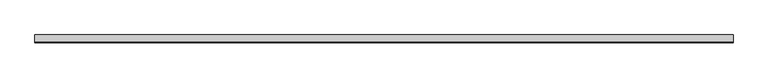
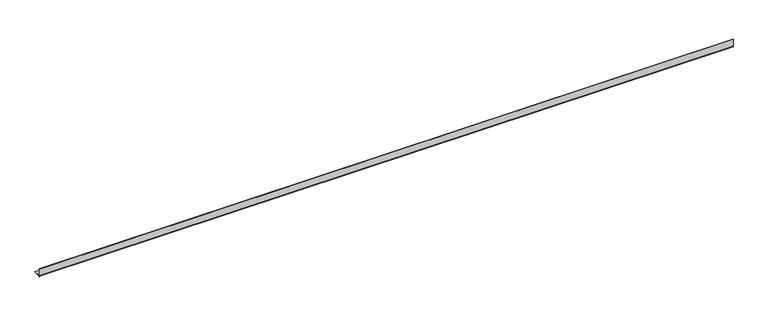
"""IFC4 building model written with IfcOpenShell, lengths in millimetres: proxy geometry, Metal profile010 3100 : Metal profile010 3100."""

import ifcopenshell
import ifcopenshell.guid

model = None  # the IFC model being written
_history = None  # IfcOwnerHistory: only IFC2X3 demands one
_inside = {}  # id of a spatial element -> (the spatial element, [elements in it])
_under = {}  # id of a project, library or spatial element -> (it, [spatial elements below it])
_declared = {}  # id of a project -> (the project, [libraries it declares])
_typed = {}  # id of a type object -> (the type object, [elements of that type])
_made_of = {}  # id of a material, layer set ... -> (it, [elements and type objects made of it])


def new_model(schema):
    """Start an empty IFC model of exactly this schema.

    Asked for "IFC4X3", IfcOpenShell would pick the latest addendum, in which some entities
    have other attributes; the version numbers below select the first issue.
    IFC2X3 requires an IfcOwnerHistory on every rooted entity: one is made here for all.
    """
    global model, _history
    if schema == "IFC4X3":
        model = ifcopenshell.file(schema_version=(4, 3, 0, 0))
    else:
        model = ifcopenshell.file(schema=schema)
    _inside.clear()
    _under.clear()
    _declared.clear()
    _typed.clear()
    _made_of.clear()
    _history = None
    if model.schema == "IFC2X3":
        org = make("IfcOrganization", Name="unknown")
        user = make(
            "IfcPersonAndOrganization",
            ThePerson=make("IfcPerson", FamilyName="unknown"),
            TheOrganization=org,
        )
        app = make(
            "IfcApplication",
            ApplicationDeveloper=org,
            Version="unknown",
            ApplicationFullName="unknown",
            ApplicationIdentifier="unknown",
        )
        _history = make(
            "IfcOwnerHistory",
            OwningUser=user,
            OwningApplication=app,
            ChangeAction="ADDED",
            CreationDate=0,
        )
    return model


def make(cls, **values):
    """One entity of the class cls with the attributes given. An attribute that is None is left unset."""
    return model.create_entity(
        cls, **{name: value for name, value in values.items() if value is not None}
    )


def rooted(cls, **values):
    """An entity with a GlobalId (a new one), such as an element, a storey or a relation."""
    return make(cls, GlobalId=ifcopenshell.guid.new(), OwnerHistory=_history, **values)


def si_unit(unit_type, name, prefix=None):
    """IfcSIUnit, for example si_unit("LENGTHUNIT", "METRE", prefix="MILLI")."""
    return make("IfcSIUnit", UnitType=unit_type, Prefix=prefix, Name=name)


def assignment(units):
    """IfcUnitAssignment: the units of a project."""
    return None if units is None else make("IfcUnitAssignment", Units=units)


def point(xyz):
    """IfcCartesianPoint."""
    return None if xyz is None else make("IfcCartesianPoint", Coordinates=xyz)


def direction(xyz):
    """IfcDirection."""
    return None if xyz is None else make("IfcDirection", DirectionRatios=xyz)


def frame(location, z_axis=None, x_axis=None):
    """IfcAxis2Placement3D, a coordinate frame: its origin and axes. An axis left out is left unset."""
    return make(
        "IfcAxis2Placement3D",
        Location=point(location),
        Axis=direction(z_axis),
        RefDirection=direction(x_axis),
    )


def frame_2d(location, x_axis=None):
    """IfcAxis2Placement2D, a coordinate frame in the plane: its origin and x axis."""
    return make(
        "IfcAxis2Placement2D", Location=point(location), RefDirection=direction(x_axis)
    )


def origin():
    """The frame at (0, 0, 0) with its axes left unset."""
    return frame((0.0, 0.0, 0.0))


def place(relative_to, where):
    """IfcLocalPlacement: puts the frame where relative to a parent placement (None: the world)."""
    return make(
        "IfcLocalPlacement", PlacementRelTo=relative_to, RelativePlacement=where
    )


def context(
    kind, dimensions, precision=None, world=None, true_north=None, identifier=None
):
    """IfcGeometricRepresentationContext, for example the 3D "Model" context."""
    return make(
        "IfcGeometricRepresentationContext",
        ContextIdentifier=identifier,
        ContextType=kind,
        CoordinateSpaceDimension=dimensions,
        Precision=precision,
        WorldCoordinateSystem=world,
        TrueNorth=true_north,
    )


def project(units=None, contexts=None):
    """IfcProject with its units and contexts."""
    return rooted(
        "IfcProject",
        Name="project",
        RepresentationContexts=contexts,
        UnitsInContext=assignment(units),
    )


def spatial(cls, under=None, at=None, **own):
    """A site, building, storey or space (cls), placed at a placement, below another one or the project."""
    s = rooted(cls, ObjectPlacement=at, **own)
    if under is not None:
        _under.setdefault(under.id(), (under, []))[1].append(s)
    return s


def polyline(points):
    """IfcPolyline through the points."""
    return make("IfcPolyline", Points=[point(p) for p in points])


def circle_curve(where, radius):
    """IfcCircle in the frame where."""
    return make("IfcCircle", Position=where, Radius=radius)


def trimmed(basis, trim1, trim2, sense, master):
    """IfcTrimmedCurve: the piece of a basis curve between two trims."""
    return make(
        "IfcTrimmedCurve",
        BasisCurve=basis,
        Trim1=trim1,
        Trim2=trim2,
        SenseAgreement=sense,
        MasterRepresentation=master,
    )


def segment(curve, same_sense, transition):
    """IfcCompositeCurveSegment."""
    return make(
        "IfcCompositeCurveSegment",
        Transition=transition,
        SameSense=same_sense,
        ParentCurve=curve,
    )


def composite_curve(segments, self_intersect=None):
    """IfcCompositeCurve: segments joined end to end."""
    return make("IfcCompositeCurve", Segments=segments, SelfIntersect=self_intersect)


def outline(outer, holes=None, kind="AREA"):
    """IfcArbitraryClosedProfileDef: a profile drawn as a closed curve; with holes, ...WithVoids."""
    if holes is None:
        return make("IfcArbitraryClosedProfileDef", ProfileType=kind, OuterCurve=outer)
    return make(
        "IfcArbitraryProfileDefWithVoids",
        ProfileType=kind,
        OuterCurve=outer,
        InnerCurves=holes,
    )


def extrude(swept, where, along, depth):
    """IfcExtrudedAreaSolid: the profile swept, set in the frame where, extruded along a direction by depth."""
    return make(
        "IfcExtrudedAreaSolid",
        SweptArea=swept,
        Position=where,
        ExtrudedDirection=direction(along),
        Depth=depth,
    )


def shape(context_of_items, identifier, shape_type, items):
    """IfcShapeRepresentation: the items that make up one representation, for example the "Body"."""
    return make(
        "IfcShapeRepresentation",
        ContextOfItems=context_of_items,
        RepresentationIdentifier=identifier,
        RepresentationType=shape_type,
        Items=items,
    )


def source(mapping_origin, context_of_items, identifier, shape_type, items):
    """IfcRepresentationMap: a shape defined once, which mapped items show again and again."""
    return make(
        "IfcRepresentationMap",
        MappingOrigin=mapping_origin,
        MappedRepresentation=shape(context_of_items, identifier, shape_type, items),
    )


def transform(
    local_origin,
    x_axis=None,
    y_axis=None,
    z_axis=None,
    scale=None,
    scale2=None,
    scale3=None,
    uniform=True,
):
    """IfcCartesianTransformationOperator3D, or its non-uniform kind. x_axis, y_axis, z_axis: its Axis1, 2, 3."""
    if uniform:
        return make(
            "IfcCartesianTransformationOperator3D",
            Axis1=direction(x_axis),
            Axis2=direction(y_axis),
            LocalOrigin=point(local_origin),
            Scale=scale,
            Axis3=direction(z_axis),
        )
    return make(
        "IfcCartesianTransformationOperator3DnonUniform",
        Axis1=direction(x_axis),
        Axis2=direction(y_axis),
        LocalOrigin=point(local_origin),
        Scale=scale,
        Axis3=direction(z_axis),
        Scale2=scale2,
        Scale3=scale3,
    )


def mapped(mapping_source, mapping_target):
    """IfcMappedItem: shows the shape of a source again, moved by a transform."""
    return make(
        "IfcMappedItem", MappingSource=mapping_source, MappingTarget=mapping_target
    )


def made_of(thing, what):
    """Note that an element or type object is made of a material, layer set ...; save() writes the relation."""
    if what is not None:
        _made_of.setdefault(what.id(), (what, []))[1].append(thing)
    return thing


def element(
    cls,
    number,
    at=None,
    inside=None,
    cuts=None,
    type_object=None,
    material=None,
    context=None,
    identifier="Body",
    shape_type=None,
    held_by="IfcProductDefinitionShape",
    body=None,
    shapes=None,
    **own,
):
    """One element of the class cls, such as IfcWall. Its Tag is "e" and its number.

    at: its placement. inside: the storey or other place that contains it. cuts: it is an
    opening in that element (IfcRelVoidsElement). A single representation is given by context,
    identifier, shape_type and body (its items); several are given by shapes. held_by: the class
    of the entity that holds the representations. save() writes the other relations.
    """
    e = rooted(cls, Tag="e%d" % number, ObjectPlacement=at, **own)
    if body is not None:
        shapes = [shape(context, identifier, shape_type, body)]
    if shapes is not None:
        e.Representation = make(held_by, Representations=shapes)
    if inside is not None:
        _inside.setdefault(inside.id(), (inside, []))[1].append(e)
    if cuts is not None:
        rooted(
            "IfcRelVoidsElement", RelatingBuildingElement=cuts, RelatedOpeningElement=e
        )
    if type_object is not None:
        _typed.setdefault(type_object.id(), (type_object, []))[1].append(e)
    return made_of(e, material)


def aggregate(whole, parts):
    """IfcRelAggregates: a whole, such as a stair, and the parts it consists of."""
    return rooted("IfcRelAggregates", RelatingObject=whole, RelatedObjects=parts)


def save(model, path):
    """Write the relations noted so far, then the file.

    IfcRelAggregates (storeys below a building ...), IfcRelContainedInSpatialStructure (elements
    in a storey), IfcRelDefinesByType, IfcRelAssociatesMaterial and IfcRelDeclares: one each for
    every whole, place, type object, material and project.
    """
    for whole, parts in _under.values():
        aggregate(whole, parts)
    for where, things in _inside.values():
        rooted(
            "IfcRelContainedInSpatialStructure",
            RelatedElements=things,
            RelatingStructure=where,
        )
    for kind, things in _typed.values():
        rooted("IfcRelDefinesByType", RelatedObjects=things, RelatingType=kind)
    for what, things in _made_of.values():
        rooted("IfcRelAssociatesMaterial", RelatedObjects=things, RelatingMaterial=what)
    for by, libraries in _declared.values():
        rooted("IfcRelDeclares", RelatingContext=by, RelatedDefinitions=libraries)
    model.write(path)


def generic_models_2c1d3a63(model_context):
    return source(origin(), model_context, "Body", "SweptSolid", [
        extrude(outline(composite_curve([segment(polyline([(10261.8870729, 42910.4253714), (10261.8870729, 42889.2721875), (10283.0402569, 42889.2721875), (10283.0402569, 42887.9921875), (10262.1373472, 42887.9921875)]), True, "CONTINUOUS"), segment(trimmed(circle_curve(frame_2d((10261.2470729, 42888.6321875)), 1.0964434), [point((10262.1373472, 42887.9921875))], [point((10260.6070729, 42889.5224617))], False, "CARTESIAN"), True, "CONTINUOUS"), segment(polyline([(10260.6070729, 42889.5224617), (10260.6070729, 42910.4253714), (10261.8870729, 42910.4253714)]), True, "CONTINUOUS")], self_intersect=False)), frame((3694.2883192, 0.0, 0.0), z_axis=(1.0, 0.0, 0.0), x_axis=(0.0, 1.0, 0.0)), (0.0, 0.0, 1.0), 2000.0),
    ])


if __name__ == "__main__":
    model = new_model("IFC4")
    model_context = context("Model", 3, world=origin())
    ifc_project = project(units=[si_unit("LENGTHUNIT", "METRE", prefix="MILLI")], contexts=[model_context])
    site = spatial("IfcSite", under=ifc_project)
    building = spatial("IfcBuilding", under=site)
    placement = place(None, origin())
    generic_models_shape = generic_models_2c1d3a63(model_context)
    element("IfcBuildingElementProxy", 1, Name="Metal profile010 3100 : Metal profile010 3100", ObjectType="Metal profile010 3100 : Metal profile010 3100", at=placement, inside=building, context=model_context, shape_type="MappedRepresentation", body=[
        mapped(generic_models_shape, transform((0.0, 0.0, 0.0), x_axis=(1.0, 0.0, 0.0), y_axis=(0.0, 1.0, 0.0), z_axis=(0.0, 0.0, 1.0))),
    ])
    save(model, "model.ifc")

# Revit data of these elements
# Type "Metal profile010 3100 : Metal profile010 3100"
#   NameOverride = "Metal profile010"
# Element 1 (IfcBuildingElementProxy, "Metal profile010 3100 : Metal profile010 3100")
#   Materials on its faces: "CORNER BEAD"
# Materials
#   "CORNER BEAD": class "Unassigned", colour RGB 255 241 0, transparency 0
